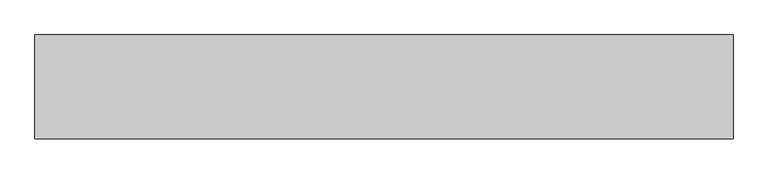
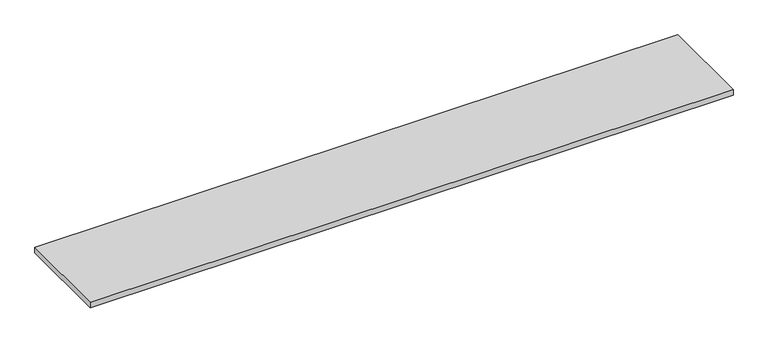
"""IFC4 building model written with IfcOpenShell, lengths in millimetres: furniture geometry, OD_CW_Countertop : OD_CW_Countertop."""

import ifcopenshell
import ifcopenshell.guid

model = None  # the IFC model being written
_history = None  # IfcOwnerHistory: only IFC2X3 demands one
_inside = {}  # id of a spatial element -> (the spatial element, [elements in it])
_under = {}  # id of a project, library or spatial element -> (it, [spatial elements below it])
_declared = {}  # id of a project -> (the project, [libraries it declares])
_typed = {}  # id of a type object -> (the type object, [elements of that type])
_made_of = {}  # id of a material, layer set ... -> (it, [elements and type objects made of it])


def new_model(schema):
    """Start an empty IFC model of exactly this schema.

    Asked for "IFC4X3", IfcOpenShell would pick the latest addendum, in which some entities
    have other attributes; the version numbers below select the first issue.
    IFC2X3 requires an IfcOwnerHistory on every rooted entity: one is made here for all.
    """
    global model, _history
    if schema == "IFC4X3":
        model = ifcopenshell.file(schema_version=(4, 3, 0, 0))
    else:
        model = ifcopenshell.file(schema=schema)
    _inside.clear()
    _under.clear()
    _declared.clear()
    _typed.clear()
    _made_of.clear()
    _history = None
    if model.schema == "IFC2X3":
        org = make("IfcOrganization", Name="unknown")
        user = make(
            "IfcPersonAndOrganization",
            ThePerson=make("IfcPerson", FamilyName="unknown"),
            TheOrganization=org,
        )
        app = make(
            "IfcApplication",
            ApplicationDeveloper=org,
            Version="unknown",
            ApplicationFullName="unknown",
            ApplicationIdentifier="unknown",
        )
        _history = make(
            "IfcOwnerHistory",
            OwningUser=user,
            OwningApplication=app,
            ChangeAction="ADDED",
            CreationDate=0,
        )
    return model


def make(cls, **values):
    """One entity of the class cls with the attributes given. An attribute that is None is left unset."""
    return model.create_entity(
        cls, **{name: value for name, value in values.items() if value is not None}
    )


def rooted(cls, **values):
    """An entity with a GlobalId (a new one), such as an element, a storey or a relation."""
    return make(cls, GlobalId=ifcopenshell.guid.new(), OwnerHistory=_history, **values)


def si_unit(unit_type, name, prefix=None):
    """IfcSIUnit, for example si_unit("LENGTHUNIT", "METRE", prefix="MILLI")."""
    return make("IfcSIUnit", UnitType=unit_type, Prefix=prefix, Name=name)


def assignment(units):
    """IfcUnitAssignment: the units of a project."""
    return None if units is None else make("IfcUnitAssignment", Units=units)


def point(xyz):
    """IfcCartesianPoint."""
    return None if xyz is None else make("IfcCartesianPoint", Coordinates=xyz)


def direction(xyz):
    """IfcDirection."""
    return None if xyz is None else make("IfcDirection", DirectionRatios=xyz)


def frame(location, z_axis=None, x_axis=None):
    """IfcAxis2Placement3D, a coordinate frame: its origin and axes. An axis left out is left unset."""
    return make(
        "IfcAxis2Placement3D",
        Location=point(location),
        Axis=direction(z_axis),
        RefDirection=direction(x_axis),
    )


def origin():
    """The frame at (0, 0, 0) with its axes left unset."""
    return frame((0.0, 0.0, 0.0))


def place(relative_to, where):
    """IfcLocalPlacement: puts the frame where relative to a parent placement (None: the world)."""
    return make(
        "IfcLocalPlacement", PlacementRelTo=relative_to, RelativePlacement=where
    )


def context(
    kind, dimensions, precision=None, world=None, true_north=None, identifier=None
):
    """IfcGeometricRepresentationContext, for example the 3D "Model" context."""
    return make(
        "IfcGeometricRepresentationContext",
        ContextIdentifier=identifier,
        ContextType=kind,
        CoordinateSpaceDimension=dimensions,
        Precision=precision,
        WorldCoordinateSystem=world,
        TrueNorth=true_north,
    )


def project(units=None, contexts=None):
    """IfcProject with its units and contexts."""
    return rooted(
        "IfcProject",
        Name="project",
        RepresentationContexts=contexts,
        UnitsInContext=assignment(units),
    )


def spatial(cls, under=None, at=None, **own):
    """A site, building, storey or space (cls), placed at a placement, below another one or the project."""
    s = rooted(cls, ObjectPlacement=at, **own)
    if under is not None:
        _under.setdefault(under.id(), (under, []))[1].append(s)
    return s


def polyline(points):
    """IfcPolyline through the points."""
    return make("IfcPolyline", Points=[point(p) for p in points])


def outline(outer, holes=None, kind="AREA"):
    """IfcArbitraryClosedProfileDef: a profile drawn as a closed curve; with holes, ...WithVoids."""
    if holes is None:
        return make("IfcArbitraryClosedProfileDef", ProfileType=kind, OuterCurve=outer)
    return make(
        "IfcArbitraryProfileDefWithVoids",
        ProfileType=kind,
        OuterCurve=outer,
        InnerCurves=holes,
    )


def extrude(swept, where, along, depth):
    """IfcExtrudedAreaSolid: the profile swept, set in the frame where, extruded along a direction by depth."""
    return make(
        "IfcExtrudedAreaSolid",
        SweptArea=swept,
        Position=where,
        ExtrudedDirection=direction(along),
        Depth=depth,
    )


def shape(context_of_items, identifier, shape_type, items):
    """IfcShapeRepresentation: the items that make up one representation, for example the "Body"."""
    return make(
        "IfcShapeRepresentation",
        ContextOfItems=context_of_items,
        RepresentationIdentifier=identifier,
        RepresentationType=shape_type,
        Items=items,
    )


def source(mapping_origin, context_of_items, identifier, shape_type, items):
    """IfcRepresentationMap: a shape defined once, which mapped items show again and again."""
    return make(
        "IfcRepresentationMap",
        MappingOrigin=mapping_origin,
        MappedRepresentation=shape(context_of_items, identifier, shape_type, items),
    )


def transform(
    local_origin,
    x_axis=None,
    y_axis=None,
    z_axis=None,
    scale=None,
    scale2=None,
    scale3=None,
    uniform=True,
):
    """IfcCartesianTransformationOperator3D, or its non-uniform kind. x_axis, y_axis, z_axis: its Axis1, 2, 3."""
    if uniform:
        return make(
            "IfcCartesianTransformationOperator3D",
            Axis1=direction(x_axis),
            Axis2=direction(y_axis),
            LocalOrigin=point(local_origin),
            Scale=scale,
            Axis3=direction(z_axis),
        )
    return make(
        "IfcCartesianTransformationOperator3DnonUniform",
        Axis1=direction(x_axis),
        Axis2=direction(y_axis),
        LocalOrigin=point(local_origin),
        Scale=scale,
        Axis3=direction(z_axis),
        Scale2=scale2,
        Scale3=scale3,
    )


def mapped(mapping_source, mapping_target):
    """IfcMappedItem: shows the shape of a source again, moved by a transform."""
    return make(
        "IfcMappedItem", MappingSource=mapping_source, MappingTarget=mapping_target
    )


def made_of(thing, what):
    """Note that an element or type object is made of a material, layer set ...; save() writes the relation."""
    if what is not None:
        _made_of.setdefault(what.id(), (what, []))[1].append(thing)
    return thing


def element(
    cls,
    number,
    at=None,
    inside=None,
    cuts=None,
    type_object=None,
    material=None,
    context=None,
    identifier="Body",
    shape_type=None,
    held_by="IfcProductDefinitionShape",
    body=None,
    shapes=None,
    **own,
):
    """One element of the class cls, such as IfcWall. Its Tag is "e" and its number.

    at: its placement. inside: the storey or other place that contains it. cuts: it is an
    opening in that element (IfcRelVoidsElement). A single representation is given by context,
    identifier, shape_type and body (its items); several are given by shapes. held_by: the class
    of the entity that holds the representations. save() writes the other relations.
    """
    e = rooted(cls, Tag="e%d" % number, ObjectPlacement=at, **own)
    if body is not None:
        shapes = [shape(context, identifier, shape_type, body)]
    if shapes is not None:
        e.Representation = make(held_by, Representations=shapes)
    if inside is not None:
        _inside.setdefault(inside.id(), (inside, []))[1].append(e)
    if cuts is not None:
        rooted(
            "IfcRelVoidsElement", RelatingBuildingElement=cuts, RelatedOpeningElement=e
        )
    if type_object is not None:
        _typed.setdefault(type_object.id(), (type_object, []))[1].append(e)
    return made_of(e, material)


def aggregate(whole, parts):
    """IfcRelAggregates: a whole, such as a stair, and the parts it consists of."""
    return rooted("IfcRelAggregates", RelatingObject=whole, RelatedObjects=parts)


def save(model, path):
    """Write the relations noted so far, then the file.

    IfcRelAggregates (storeys below a building ...), IfcRelContainedInSpatialStructure (elements
    in a storey), IfcRelDefinesByType, IfcRelAssociatesMaterial and IfcRelDeclares: one each for
    every whole, place, type object, material and project.
    """
    for whole, parts in _under.values():
        aggregate(whole, parts)
    for where, things in _inside.values():
        rooted(
            "IfcRelContainedInSpatialStructure",
            RelatedElements=things,
            RelatingStructure=where,
        )
    for kind, things in _typed.values():
        rooted("IfcRelDefinesByType", RelatedObjects=things, RelatingType=kind)
    for what, things in _made_of.values():
        rooted("IfcRelAssociatesMaterial", RelatedObjects=things, RelatingMaterial=what)
    for by, libraries in _declared.values():
        rooted("IfcRelDeclares", RelatingContext=by, RelatedDefinitions=libraries)
    model.write(path)


def furniture_75740181(model_context):
    return source(origin(), model_context, "Body", "SweptSolid", [
        extrude(outline(polyline([(18.7377049, -609.6), (18.7377049, 25.4), (4285.9377049, 25.4), (4285.9377049, -609.6), (18.7377049, -609.6)])), frame((0.0, 0.0, 965.2), z_axis=(0.0, 0.0, 1.0), x_axis=(1.0, 0.0, 0.0)), (0.0, 0.0, 1.0), 38.1),
    ])


if __name__ == "__main__":
    model = new_model("IFC4")
    model_context = context("Model", 3, world=origin())
    ifc_project = project(units=[si_unit("LENGTHUNIT", "METRE", prefix="MILLI")], contexts=[model_context])
    site = spatial("IfcSite", under=ifc_project)
    building = spatial("IfcBuilding", under=site)
    placement = place(None, origin())
    furniture_shape = furniture_75740181(model_context)
    element("IfcFurniture", 1, ObjectType="OD_CW_Countertop : OD_CW_Countertop", at=placement, inside=building, context=model_context, shape_type="MappedRepresentation", body=[
        mapped(furniture_shape, transform((0.0, 0.0, 0.0), x_axis=(1.0, 0.0, 0.0), y_axis=(0.0, 1.0, 0.0), z_axis=(0.0, 0.0, 1.0))),
    ])
    save(model, "model.ifc")

# Revit data of these elements
# Type "OD_CW_Countertop : OD_CW_Countertop"
#   OD_CW_Width [instance default] = 2' - 9"
#   OD_CW_Off Floor [instance default] = 3' - 2"
#   OD_CW_Length [instance default] = 6' - 9"
#   OD_CW_Height [instance default] = 7' - 0"
#   Depth = 2' - 0"
#   Height = 3' - 0"
#   Width = 4' - 0"
#   OD_CW_Material_Countertop [instance default] = none
# Element 1 (IfcFurniture, "OD_CW_Countertop : OD_CW_Countertop")
#   OD_CW_Width = 2' - 1"
#   OD_CW_Length = 14' - 0"
#   OD_CW_Height = 0' - 1 1/2"
#   Materials on its faces: "CASEWORK"
# Materials
#   "CASEWORK": class "Generic", colour RGB 181 181 181, transparency 0, Cost = 0
